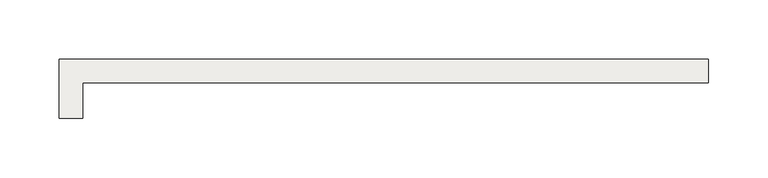
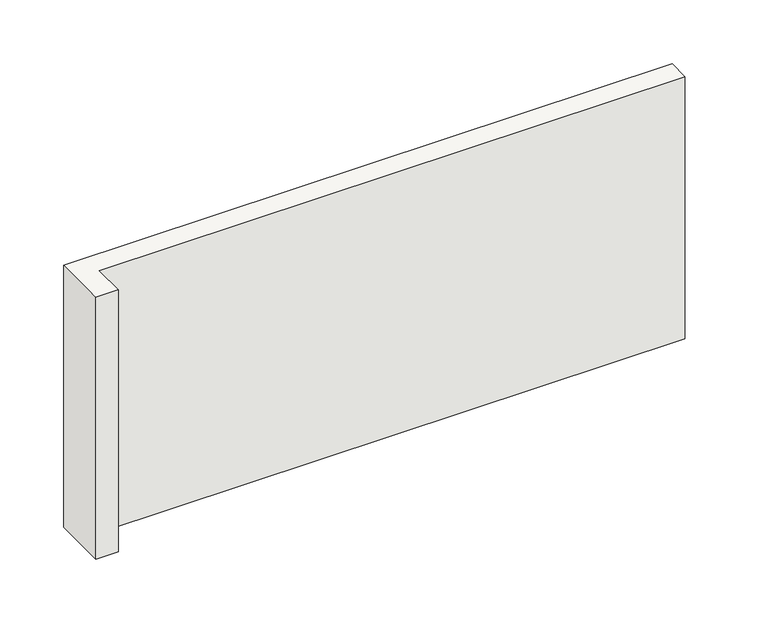
"""IFC4 building model written with IfcOpenShell, lengths in millimetres: slab geometry, FECHAMENTO DECK DE MADEIRA - PATAMAR ENTRADA 1 : FECHAMENTO DECK DE MADEIRA - PATAMAR ENTRADA 2."""

import ifcopenshell
import ifcopenshell.guid

model = None  # the IFC model being written
_history = None  # IfcOwnerHistory: only IFC2X3 demands one
_inside = {}  # id of a spatial element -> (the spatial element, [elements in it])
_under = {}  # id of a project, library or spatial element -> (it, [spatial elements below it])
_declared = {}  # id of a project -> (the project, [libraries it declares])
_typed = {}  # id of a type object -> (the type object, [elements of that type])
_made_of = {}  # id of a material, layer set ... -> (it, [elements and type objects made of it])


def new_model(schema):
    """Start an empty IFC model of exactly this schema.

    Asked for "IFC4X3", IfcOpenShell would pick the latest addendum, in which some entities
    have other attributes; the version numbers below select the first issue.
    IFC2X3 requires an IfcOwnerHistory on every rooted entity: one is made here for all.
    """
    global model, _history
    if schema == "IFC4X3":
        model = ifcopenshell.file(schema_version=(4, 3, 0, 0))
    else:
        model = ifcopenshell.file(schema=schema)
    _inside.clear()
    _under.clear()
    _declared.clear()
    _typed.clear()
    _made_of.clear()
    _history = None
    if model.schema == "IFC2X3":
        org = make("IfcOrganization", Name="unknown")
        user = make(
            "IfcPersonAndOrganization",
            ThePerson=make("IfcPerson", FamilyName="unknown"),
            TheOrganization=org,
        )
        app = make(
            "IfcApplication",
            ApplicationDeveloper=org,
            Version="unknown",
            ApplicationFullName="unknown",
            ApplicationIdentifier="unknown",
        )
        _history = make(
            "IfcOwnerHistory",
            OwningUser=user,
            OwningApplication=app,
            ChangeAction="ADDED",
            CreationDate=0,
        )
    return model


def make(cls, **values):
    """One entity of the class cls with the attributes given. An attribute that is None is left unset."""
    return model.create_entity(
        cls, **{name: value for name, value in values.items() if value is not None}
    )


def rooted(cls, **values):
    """An entity with a GlobalId (a new one), such as an element, a storey or a relation."""
    return make(cls, GlobalId=ifcopenshell.guid.new(), OwnerHistory=_history, **values)


def si_unit(unit_type, name, prefix=None):
    """IfcSIUnit, for example si_unit("LENGTHUNIT", "METRE", prefix="MILLI")."""
    return make("IfcSIUnit", UnitType=unit_type, Prefix=prefix, Name=name)


def assignment(units):
    """IfcUnitAssignment: the units of a project."""
    return None if units is None else make("IfcUnitAssignment", Units=units)


def point(xyz):
    """IfcCartesianPoint."""
    return None if xyz is None else make("IfcCartesianPoint", Coordinates=xyz)


def direction(xyz):
    """IfcDirection."""
    return None if xyz is None else make("IfcDirection", DirectionRatios=xyz)


def frame(location, z_axis=None, x_axis=None):
    """IfcAxis2Placement3D, a coordinate frame: its origin and axes. An axis left out is left unset."""
    return make(
        "IfcAxis2Placement3D",
        Location=point(location),
        Axis=direction(z_axis),
        RefDirection=direction(x_axis),
    )


def origin():
    """The frame at (0, 0, 0) with its axes left unset."""
    return frame((0.0, 0.0, 0.0))


def place(relative_to, where):
    """IfcLocalPlacement: puts the frame where relative to a parent placement (None: the world)."""
    return make(
        "IfcLocalPlacement", PlacementRelTo=relative_to, RelativePlacement=where
    )


def context(
    kind, dimensions, precision=None, world=None, true_north=None, identifier=None
):
    """IfcGeometricRepresentationContext, for example the 3D "Model" context."""
    return make(
        "IfcGeometricRepresentationContext",
        ContextIdentifier=identifier,
        ContextType=kind,
        CoordinateSpaceDimension=dimensions,
        Precision=precision,
        WorldCoordinateSystem=world,
        TrueNorth=true_north,
    )


def project(units=None, contexts=None):
    """IfcProject with its units and contexts."""
    return rooted(
        "IfcProject",
        Name="project",
        RepresentationContexts=contexts,
        UnitsInContext=assignment(units),
    )


def spatial(cls, under=None, at=None, **own):
    """A site, building, storey or space (cls), placed at a placement, below another one or the project."""
    s = rooted(cls, ObjectPlacement=at, **own)
    if under is not None:
        _under.setdefault(under.id(), (under, []))[1].append(s)
    return s


def polyline(points):
    """IfcPolyline through the points."""
    return make("IfcPolyline", Points=[point(p) for p in points])


def outline(outer, holes=None, kind="AREA"):
    """IfcArbitraryClosedProfileDef: a profile drawn as a closed curve; with holes, ...WithVoids."""
    if holes is None:
        return make("IfcArbitraryClosedProfileDef", ProfileType=kind, OuterCurve=outer)
    return make(
        "IfcArbitraryProfileDefWithVoids",
        ProfileType=kind,
        OuterCurve=outer,
        InnerCurves=holes,
    )


def extrude(swept, where, along, depth):
    """IfcExtrudedAreaSolid: the profile swept, set in the frame where, extruded along a direction by depth."""
    return make(
        "IfcExtrudedAreaSolid",
        SweptArea=swept,
        Position=where,
        ExtrudedDirection=direction(along),
        Depth=depth,
    )


def shape(context_of_items, identifier, shape_type, items):
    """IfcShapeRepresentation: the items that make up one representation, for example the "Body"."""
    return make(
        "IfcShapeRepresentation",
        ContextOfItems=context_of_items,
        RepresentationIdentifier=identifier,
        RepresentationType=shape_type,
        Items=items,
    )


def source(mapping_origin, context_of_items, identifier, shape_type, items):
    """IfcRepresentationMap: a shape defined once, which mapped items show again and again."""
    return make(
        "IfcRepresentationMap",
        MappingOrigin=mapping_origin,
        MappedRepresentation=shape(context_of_items, identifier, shape_type, items),
    )


def transform(
    local_origin,
    x_axis=None,
    y_axis=None,
    z_axis=None,
    scale=None,
    scale2=None,
    scale3=None,
    uniform=True,
):
    """IfcCartesianTransformationOperator3D, or its non-uniform kind. x_axis, y_axis, z_axis: its Axis1, 2, 3."""
    if uniform:
        return make(
            "IfcCartesianTransformationOperator3D",
            Axis1=direction(x_axis),
            Axis2=direction(y_axis),
            LocalOrigin=point(local_origin),
            Scale=scale,
            Axis3=direction(z_axis),
        )
    return make(
        "IfcCartesianTransformationOperator3DnonUniform",
        Axis1=direction(x_axis),
        Axis2=direction(y_axis),
        LocalOrigin=point(local_origin),
        Scale=scale,
        Axis3=direction(z_axis),
        Scale2=scale2,
        Scale3=scale3,
    )


def mapped(mapping_source, mapping_target):
    """IfcMappedItem: shows the shape of a source again, moved by a transform."""
    return make(
        "IfcMappedItem", MappingSource=mapping_source, MappingTarget=mapping_target
    )


def made_of(thing, what):
    """Note that an element or type object is made of a material, layer set ...; save() writes the relation."""
    if what is not None:
        _made_of.setdefault(what.id(), (what, []))[1].append(thing)
    return thing


def element(
    cls,
    number,
    at=None,
    inside=None,
    cuts=None,
    type_object=None,
    material=None,
    context=None,
    identifier="Body",
    shape_type=None,
    held_by="IfcProductDefinitionShape",
    body=None,
    shapes=None,
    **own,
):
    """One element of the class cls, such as IfcWall. Its Tag is "e" and its number.

    at: its placement. inside: the storey or other place that contains it. cuts: it is an
    opening in that element (IfcRelVoidsElement). A single representation is given by context,
    identifier, shape_type and body (its items); several are given by shapes. held_by: the class
    of the entity that holds the representations. save() writes the other relations.
    """
    e = rooted(cls, Tag="e%d" % number, ObjectPlacement=at, **own)
    if body is not None:
        shapes = [shape(context, identifier, shape_type, body)]
    if shapes is not None:
        e.Representation = make(held_by, Representations=shapes)
    if inside is not None:
        _inside.setdefault(inside.id(), (inside, []))[1].append(e)
    if cuts is not None:
        rooted(
            "IfcRelVoidsElement", RelatingBuildingElement=cuts, RelatedOpeningElement=e
        )
    if type_object is not None:
        _typed.setdefault(type_object.id(), (type_object, []))[1].append(e)
    return made_of(e, material)


def aggregate(whole, parts):
    """IfcRelAggregates: a whole, such as a stair, and the parts it consists of."""
    return rooted("IfcRelAggregates", RelatingObject=whole, RelatedObjects=parts)


def save(model, path):
    """Write the relations noted so far, then the file.

    IfcRelAggregates (storeys below a building ...), IfcRelContainedInSpatialStructure (elements
    in a storey), IfcRelDefinesByType, IfcRelAssociatesMaterial and IfcRelDeclares: one each for
    every whole, place, type object, material and project.
    """
    for whole, parts in _under.values():
        aggregate(whole, parts)
    for where, things in _inside.values():
        rooted(
            "IfcRelContainedInSpatialStructure",
            RelatedElements=things,
            RelatingStructure=where,
        )
    for kind, things in _typed.values():
        rooted("IfcRelDefinesByType", RelatedObjects=things, RelatingType=kind)
    for what, things in _made_of.values():
        rooted("IfcRelAssociatesMaterial", RelatedObjects=things, RelatingMaterial=what)
    for by, libraries in _declared.values():
        rooted("IfcRelDeclares", RelatingContext=by, RelatedDefinitions=libraries)
    model.write(path)


def slab_ac09833d(model_context):
    return source(origin(), model_context, "Body", "SweptSolid", [
        extrude(outline(polyline([(-7189.281307, -2045.5699847), (-7209.281307, -2045.5699847), (-7209.281307, -1995.5699847), (-6660.281307, -1995.5699847), (-6660.281307, -2015.5699847), (-7189.281307, -2015.5699847), (-7189.281307, -2045.5699847)])), frame((0.0, 0.0, 80.0), z_axis=(0.0, 0.0, 1.0), x_axis=(1.0, 0.0, 0.0)), (0.0, 0.0, 1.0), 250.0),
    ])


if __name__ == "__main__":
    model = new_model("IFC4")
    model_context = context("Model", 3, world=origin())
    ifc_project = project(units=[si_unit("LENGTHUNIT", "METRE", prefix="MILLI")], contexts=[model_context])
    site = spatial("IfcSite", under=ifc_project)
    building = spatial("IfcBuilding", under=site)
    placement = place(None, origin())
    slab_shape = slab_ac09833d(model_context)
    element("IfcSlab", 1, ObjectType="FECHAMENTO DECK DE MADEIRA - PATAMAR ENTRADA 1 : FECHAMENTO DECK DE MADEIRA - PATAMAR ENTRADA 2", at=placement, inside=building, context=model_context, shape_type="MappedRepresentation", body=[
        mapped(slab_shape, transform((0.0, 0.0, 0.0), x_axis=(1.0, 0.0, 0.0), y_axis=(0.0, 1.0, 0.0), z_axis=(0.0, 0.0, 1.0))),
    ])
    save(model, "model.ifc")

# Revit data of these elements
# Element 1 (IfcSlab, "FECHAMENTO DECK DE MADEIRA - PATAMAR ENTRADA 1 : FECHAMENTO DECK DE MADEIRA - PATAMAR ENTRADA 2")
#   Materials on its faces: ".DECK DE MADEIRA TRANSVERSAL"
# Materials
#   ".DECK DE MADEIRA TRANSVERSAL": class ".CC_MADEIRA REVEST.", colour RGB 169 114 85, transparency 0, Description = "Deck de madeira", Cost = 0
